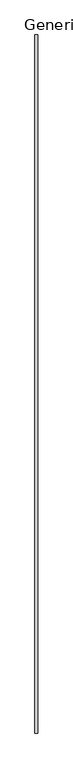
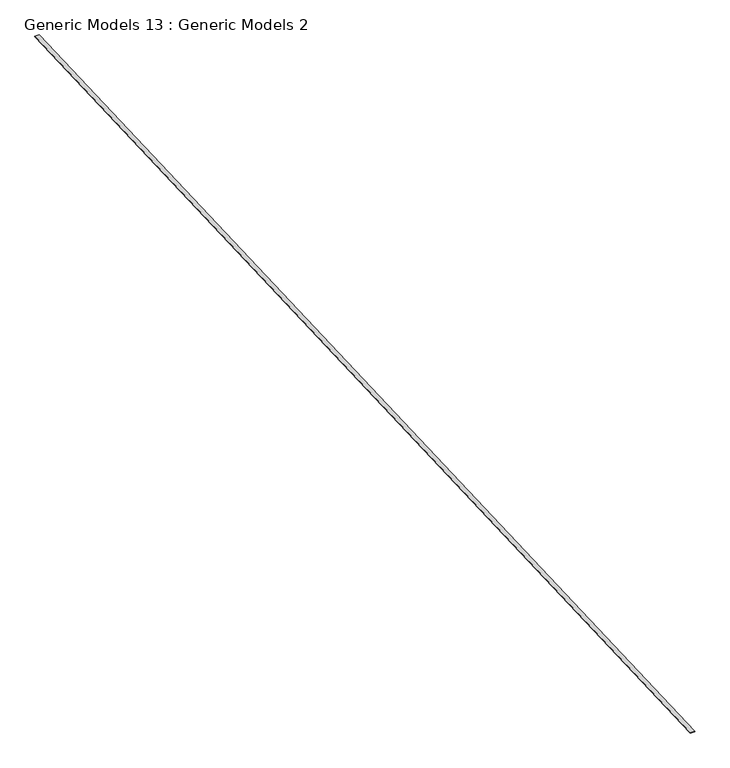
"""IFC4 building model written with IfcOpenShell, lengths in millimetres: proxy geometry, Generic Models 13 : Generic Models 2."""

from ifc_helpers import new_model, si_unit, frame, origin, place, context, project, spatial, polyline, outline, extrude, source, transform, mapped, element, save


def generic_models_13_generic_models_2_99645d9e(model_context):
    return source(origin(), model_context, "Body", "SweptSolid", [
        extrude(outline(polyline([(0.0, -130.2686535), (0.0, 0.0), (33406.7702703, 0.0), (33406.7702703, -130.2686535), (0.0, -130.2686535)])), frame((667475.506668, -569978.7590519, 8776.8517411), z_axis=(0.0, -0.041630544712176865, 0.9991330730923521), x_axis=(0.0, 0.9991330730923521, 0.041630544712176865)), (0.0, 0.0, 1.0), 4.7625),
    ])


if __name__ == "__main__":
    model = new_model("IFC4")
    model_context = context("Model", 3, world=origin())
    ifc_project = project(units=[si_unit("LENGTHUNIT", "METRE", prefix="MILLI")], contexts=[model_context])
    site = spatial("IfcSite", under=ifc_project)
    building = spatial("IfcBuilding", under=site)
    placement = place(None, origin())
    generic_models_13_generic_models_2_shape = generic_models_13_generic_models_2_99645d9e(model_context)
    element("IfcBuildingElementProxy", 1, Name="Generic Models 13 : Generic Models 2", ObjectType="Generic Models 13 : Generic Models 2", at=placement, inside=building, context=model_context, shape_type="MappedRepresentation", body=[
        mapped(generic_models_13_generic_models_2_shape, transform((0.0, 0.0, 0.0), x_axis=(1.0, 0.0, 0.0), y_axis=(0.0, 1.0, 0.0), z_axis=(0.0, 0.0, 1.0))),
    ])
    save(model, "model.ifc")

# Revit data of these elements
# Element 1 (IfcBuildingElementProxy, "Generic Models 13 : Generic Models 2")
#   Materials on its faces: "STEEL PLATE FOR STOREFRONT SUPPORT T.B.D."
# Materials
#   "STEEL PLATE FOR STOREFRONT SUPPORT T.B.D.": class "Metal", colour RGB 189 187 185, transparency 0, Description = "Structural steel 50ksi", Cost = 0
